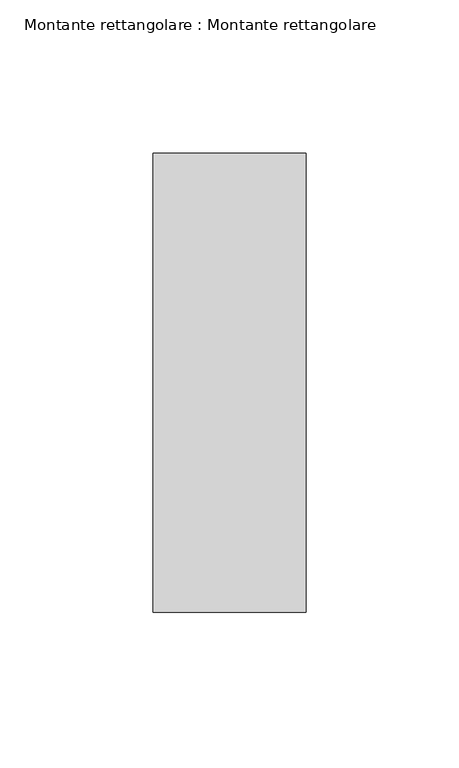
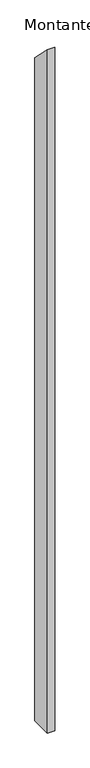
"""IFC4 building model written with IfcOpenShell, lengths in millimetres: member geometry, Montante rettangolare : Montante rettangolare."""

from ifc_helpers import new_model, si_unit, frame, origin, place, context, project, spatial, polyline, outline, extrude, source, transform, mapped, element, save


def montante_rettangolare_montante_rettangolare_efcb39a4(model_context):
    return source(origin(), model_context, "Body", "SweptSolid", [
        extrude(outline(polyline([(-75.0, 75.0), (75.0, -75.0), (75.0, -4920.0), (-75.0, -4920.0), (-75.0, 75.0)])), frame((-50.0, 0.0, 0.0), z_axis=(1.0, 0.0, 0.0), x_axis=(0.0, 1.0, 0.0)), (0.0, 0.0, 1.0), 50.0),
    ])


if __name__ == "__main__":
    model = new_model("IFC4")
    model_context = context("Model", 3, world=origin())
    ifc_project = project(units=[si_unit("LENGTHUNIT", "METRE", prefix="MILLI")], contexts=[model_context])
    site = spatial("IfcSite", under=ifc_project)
    building = spatial("IfcBuilding", under=site)
    placement = place(None, origin())
    montante_rettangolare_montante_rettangolare_shape = montante_rettangolare_montante_rettangolare_efcb39a4(model_context)
    element("IfcMember", 1, ObjectType="Montante rettangolare : Montante rettangolare", at=placement, inside=building, context=model_context, shape_type="MappedRepresentation", body=[
        mapped(montante_rettangolare_montante_rettangolare_shape, transform((0.0, 0.0, 0.0), x_axis=(1.0, 0.0, 0.0), y_axis=(0.0, 1.0, 0.0), z_axis=(0.0, 0.0, 1.0))),
    ])
    save(model, "model.ifc")

# Revit data of these elements
# Type "Montante rettangolare : Montante rettangolare"
#   built-in parameter 1007304 = 0.492126 (stored number, unit not read)
#   built-in parameter 1007301 = 0.082021 (stored number, unit not read)
#   built-in parameter 1007300 = 0.082021 (stored number, unit not read)
# Element 1 (IfcMember, "Montante rettangolare : Montante rettangolare")
#   Materials on its faces: "Acciaio"
# Materials
#   "Acciaio": class "Metallo", colour RGB 247 247 247, transparency 0, Description = "Acciaio, finitura zigrinata", Cost = 0
